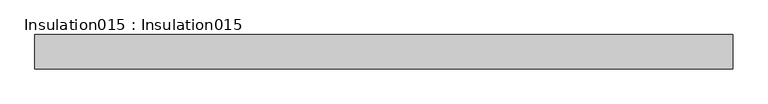
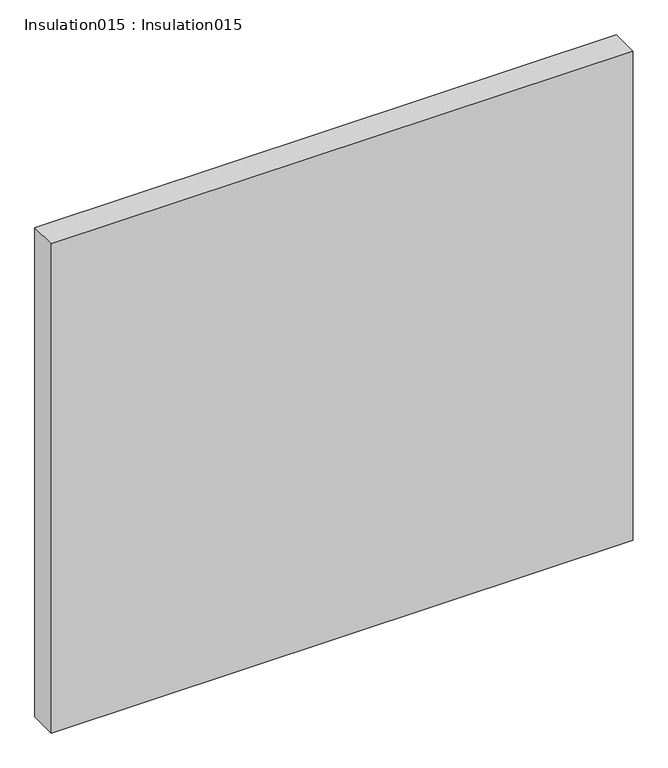
"""IFC4 building model written with IfcOpenShell, lengths in millimetres: proxy geometry, Insulation015 : Insulation015."""

from ifc_helpers import new_model, si_unit, frame, origin, place, context, project, spatial, polyline, outline, extrude, source, transform, mapped, element, save


def insulation015_insulation015_96dce9c3(model_context):
    return source(origin(), model_context, "Body", "SweptSolid", [
        extrude(outline(polyline([(12383.0178845, -4623.3867188), (12383.0178845, -4524.8317946), (14383.0178845, -4524.8317946), (14383.0178845, -4623.3867188), (12383.0178845, -4623.3867188)])), frame((0.0, 0.0, 36582.096), z_axis=(0.0, 0.0, 1.0), x_axis=(1.0, 0.0, 0.0)), (0.0, 0.0, 1.0), 1778.0016562),
    ])


if __name__ == "__main__":
    model = new_model("IFC4")
    model_context = context("Model", 3, world=origin())
    ifc_project = project(units=[si_unit("LENGTHUNIT", "METRE", prefix="MILLI")], contexts=[model_context])
    site = spatial("IfcSite", under=ifc_project)
    building = spatial("IfcBuilding", under=site)
    placement = place(None, origin())
    insulation015_insulation015_shape = insulation015_insulation015_96dce9c3(model_context)
    element("IfcBuildingElementProxy", 1, Name="Insulation015 : Insulation015", ObjectType="Insulation015 : Insulation015", at=placement, inside=building, context=model_context, shape_type="MappedRepresentation", body=[
        mapped(insulation015_insulation015_shape, transform((0.0, 0.0, 0.0), x_axis=(1.0, 0.0, 0.0), y_axis=(0.0, 1.0, 0.0), z_axis=(0.0, 0.0, 1.0))),
    ])
    save(model, "model.ifc")

# Revit data of these elements
# Type "Insulation015 : Insulation015"
#   NameOverride = "Insulation015"
# Element 1 (IfcBuildingElementProxy, "Insulation015 : Insulation015")
#   Materials on its faces: "BATT INSULATION (U-FACTOR = 0.065 MIN.) OVER CLASS II VAPOR RETARDER (TOWARDS INTERIOR)"
# Materials
#   "BATT INSULATION (U-FACTOR = 0.065 MIN.) OVER CLASS II VAPOR RETARDER (TOWARDS INTERIOR)": class "Unassigned", colour RGB 246 242 160, transparency 0, Cost = 0
